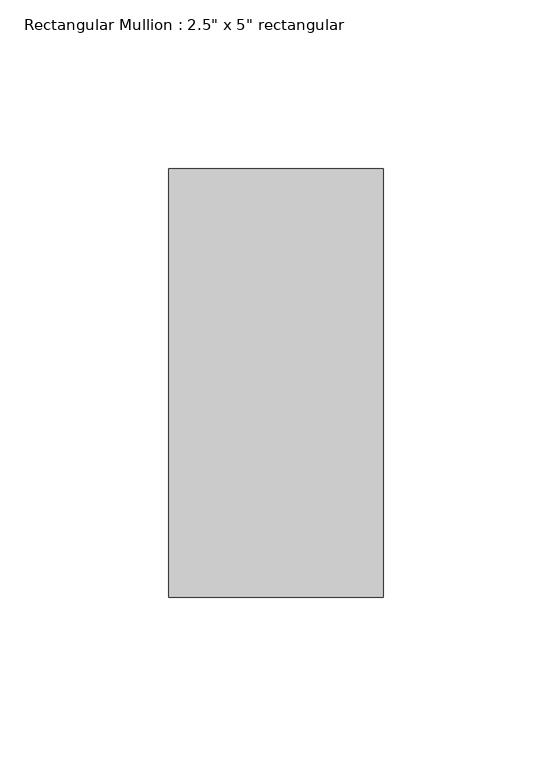
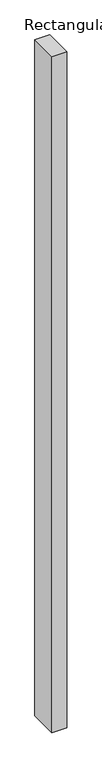
"""IFC4 building model written with IfcOpenShell, lengths in millimetres: member geometry."""

import ifcopenshell
import ifcopenshell.guid

model = None  # the IFC model being written
_history = None  # IfcOwnerHistory: only IFC2X3 demands one
_inside = {}  # id of a spatial element -> (the spatial element, [elements in it])
_under = {}  # id of a project, library or spatial element -> (it, [spatial elements below it])
_declared = {}  # id of a project -> (the project, [libraries it declares])
_typed = {}  # id of a type object -> (the type object, [elements of that type])
_made_of = {}  # id of a material, layer set ... -> (it, [elements and type objects made of it])


def new_model(schema):
    """Start an empty IFC model of exactly this schema.

    Asked for "IFC4X3", IfcOpenShell would pick the latest addendum, in which some entities
    have other attributes; the version numbers below select the first issue.
    IFC2X3 requires an IfcOwnerHistory on every rooted entity: one is made here for all.
    """
    global model, _history
    if schema == "IFC4X3":
        model = ifcopenshell.file(schema_version=(4, 3, 0, 0))
    else:
        model = ifcopenshell.file(schema=schema)
    _inside.clear()
    _under.clear()
    _declared.clear()
    _typed.clear()
    _made_of.clear()
    _history = None
    if model.schema == "IFC2X3":
        org = make("IfcOrganization", Name="unknown")
        user = make(
            "IfcPersonAndOrganization",
            ThePerson=make("IfcPerson", FamilyName="unknown"),
            TheOrganization=org,
        )
        app = make(
            "IfcApplication",
            ApplicationDeveloper=org,
            Version="unknown",
            ApplicationFullName="unknown",
            ApplicationIdentifier="unknown",
        )
        _history = make(
            "IfcOwnerHistory",
            OwningUser=user,
            OwningApplication=app,
            ChangeAction="ADDED",
            CreationDate=0,
        )
    return model


def make(cls, **values):
    """One entity of the class cls with the attributes given. An attribute that is None is left unset."""
    return model.create_entity(
        cls, **{name: value for name, value in values.items() if value is not None}
    )


def rooted(cls, **values):
    """An entity with a GlobalId (a new one), such as an element, a storey or a relation."""
    return make(cls, GlobalId=ifcopenshell.guid.new(), OwnerHistory=_history, **values)


def si_unit(unit_type, name, prefix=None):
    """IfcSIUnit, for example si_unit("LENGTHUNIT", "METRE", prefix="MILLI")."""
    return make("IfcSIUnit", UnitType=unit_type, Prefix=prefix, Name=name)


def assignment(units):
    """IfcUnitAssignment: the units of a project."""
    return None if units is None else make("IfcUnitAssignment", Units=units)


def point(xyz):
    """IfcCartesianPoint."""
    return None if xyz is None else make("IfcCartesianPoint", Coordinates=xyz)


def direction(xyz):
    """IfcDirection."""
    return None if xyz is None else make("IfcDirection", DirectionRatios=xyz)


def frame(location, z_axis=None, x_axis=None):
    """IfcAxis2Placement3D, a coordinate frame: its origin and axes. An axis left out is left unset."""
    return make(
        "IfcAxis2Placement3D",
        Location=point(location),
        Axis=direction(z_axis),
        RefDirection=direction(x_axis),
    )


def origin():
    """The frame at (0, 0, 0) with its axes left unset."""
    return frame((0.0, 0.0, 0.0))


def place(relative_to, where):
    """IfcLocalPlacement: puts the frame where relative to a parent placement (None: the world)."""
    return make(
        "IfcLocalPlacement", PlacementRelTo=relative_to, RelativePlacement=where
    )


def context(
    kind, dimensions, precision=None, world=None, true_north=None, identifier=None
):
    """IfcGeometricRepresentationContext, for example the 3D "Model" context."""
    return make(
        "IfcGeometricRepresentationContext",
        ContextIdentifier=identifier,
        ContextType=kind,
        CoordinateSpaceDimension=dimensions,
        Precision=precision,
        WorldCoordinateSystem=world,
        TrueNorth=true_north,
    )


def project(units=None, contexts=None):
    """IfcProject with its units and contexts."""
    return rooted(
        "IfcProject",
        Name="project",
        RepresentationContexts=contexts,
        UnitsInContext=assignment(units),
    )


def spatial(cls, under=None, at=None, **own):
    """A site, building, storey or space (cls), placed at a placement, below another one or the project."""
    s = rooted(cls, ObjectPlacement=at, **own)
    if under is not None:
        _under.setdefault(under.id(), (under, []))[1].append(s)
    return s


def polyline(points):
    """IfcPolyline through the points."""
    return make("IfcPolyline", Points=[point(p) for p in points])


def outline(outer, holes=None, kind="AREA"):
    """IfcArbitraryClosedProfileDef: a profile drawn as a closed curve; with holes, ...WithVoids."""
    if holes is None:
        return make("IfcArbitraryClosedProfileDef", ProfileType=kind, OuterCurve=outer)
    return make(
        "IfcArbitraryProfileDefWithVoids",
        ProfileType=kind,
        OuterCurve=outer,
        InnerCurves=holes,
    )


def extrude(swept, where, along, depth):
    """IfcExtrudedAreaSolid: the profile swept, set in the frame where, extruded along a direction by depth."""
    return make(
        "IfcExtrudedAreaSolid",
        SweptArea=swept,
        Position=where,
        ExtrudedDirection=direction(along),
        Depth=depth,
    )


def shape(context_of_items, identifier, shape_type, items):
    """IfcShapeRepresentation: the items that make up one representation, for example the "Body"."""
    return make(
        "IfcShapeRepresentation",
        ContextOfItems=context_of_items,
        RepresentationIdentifier=identifier,
        RepresentationType=shape_type,
        Items=items,
    )


def source(mapping_origin, context_of_items, identifier, shape_type, items):
    """IfcRepresentationMap: a shape defined once, which mapped items show again and again."""
    return make(
        "IfcRepresentationMap",
        MappingOrigin=mapping_origin,
        MappedRepresentation=shape(context_of_items, identifier, shape_type, items),
    )


def transform(
    local_origin,
    x_axis=None,
    y_axis=None,
    z_axis=None,
    scale=None,
    scale2=None,
    scale3=None,
    uniform=True,
):
    """IfcCartesianTransformationOperator3D, or its non-uniform kind. x_axis, y_axis, z_axis: its Axis1, 2, 3."""
    if uniform:
        return make(
            "IfcCartesianTransformationOperator3D",
            Axis1=direction(x_axis),
            Axis2=direction(y_axis),
            LocalOrigin=point(local_origin),
            Scale=scale,
            Axis3=direction(z_axis),
        )
    return make(
        "IfcCartesianTransformationOperator3DnonUniform",
        Axis1=direction(x_axis),
        Axis2=direction(y_axis),
        LocalOrigin=point(local_origin),
        Scale=scale,
        Axis3=direction(z_axis),
        Scale2=scale2,
        Scale3=scale3,
    )


def mapped(mapping_source, mapping_target):
    """IfcMappedItem: shows the shape of a source again, moved by a transform."""
    return make(
        "IfcMappedItem", MappingSource=mapping_source, MappingTarget=mapping_target
    )


def made_of(thing, what):
    """Note that an element or type object is made of a material, layer set ...; save() writes the relation."""
    if what is not None:
        _made_of.setdefault(what.id(), (what, []))[1].append(thing)
    return thing


def element(
    cls,
    number,
    at=None,
    inside=None,
    cuts=None,
    type_object=None,
    material=None,
    context=None,
    identifier="Body",
    shape_type=None,
    held_by="IfcProductDefinitionShape",
    body=None,
    shapes=None,
    **own,
):
    """One element of the class cls, such as IfcWall. Its Tag is "e" and its number.

    at: its placement. inside: the storey or other place that contains it. cuts: it is an
    opening in that element (IfcRelVoidsElement). A single representation is given by context,
    identifier, shape_type and body (its items); several are given by shapes. held_by: the class
    of the entity that holds the representations. save() writes the other relations.
    """
    e = rooted(cls, Tag="e%d" % number, ObjectPlacement=at, **own)
    if body is not None:
        shapes = [shape(context, identifier, shape_type, body)]
    if shapes is not None:
        e.Representation = make(held_by, Representations=shapes)
    if inside is not None:
        _inside.setdefault(inside.id(), (inside, []))[1].append(e)
    if cuts is not None:
        rooted(
            "IfcRelVoidsElement", RelatingBuildingElement=cuts, RelatedOpeningElement=e
        )
    if type_object is not None:
        _typed.setdefault(type_object.id(), (type_object, []))[1].append(e)
    return made_of(e, material)


def aggregate(whole, parts):
    """IfcRelAggregates: a whole, such as a stair, and the parts it consists of."""
    return rooted("IfcRelAggregates", RelatingObject=whole, RelatedObjects=parts)


def save(model, path):
    """Write the relations noted so far, then the file.

    IfcRelAggregates (storeys below a building ...), IfcRelContainedInSpatialStructure (elements
    in a storey), IfcRelDefinesByType, IfcRelAssociatesMaterial and IfcRelDeclares: one each for
    every whole, place, type object, material and project.
    """
    for whole, parts in _under.values():
        aggregate(whole, parts)
    for where, things in _inside.values():
        rooted(
            "IfcRelContainedInSpatialStructure",
            RelatedElements=things,
            RelatingStructure=where,
        )
    for kind, things in _typed.values():
        rooted("IfcRelDefinesByType", RelatedObjects=things, RelatingType=kind)
    for what, things in _made_of.values():
        rooted("IfcRelAssociatesMaterial", RelatedObjects=things, RelatingMaterial=what)
    for by, libraries in _declared.values():
        rooted("IfcRelDeclares", RelatingContext=by, RelatedDefinitions=libraries)
    model.write(path)


def member_e8b2a95c(model_context):
    return source(origin(), model_context, "Body", "SweptSolid", [
        extrude(outline(polyline([(0.0, 63.5), (0.0, -63.5), (-63.5, -63.5), (-63.5, 63.5), (0.0, 63.5)])), frame((0.0, 0.0, -3086.1), z_axis=(0.0, 0.0, 1.0), x_axis=(1.0, 0.0, 0.0)), (0.0, 0.0, 1.0), 3086.1),
    ])


if __name__ == "__main__":
    model = new_model("IFC4")
    model_context = context("Model", 3, world=origin())
    ifc_project = project(units=[si_unit("LENGTHUNIT", "METRE", prefix="MILLI")], contexts=[model_context])
    site = spatial("IfcSite", under=ifc_project)
    building = spatial("IfcBuilding", under=site)
    placement = place(None, origin())
    member_shape = member_e8b2a95c(model_context)
    element("IfcMember", 1, ObjectType="Rectangular Mullion : 2.5\" x 5\" rectangular", at=placement, inside=building, context=model_context, shape_type="MappedRepresentation", body=[
        mapped(member_shape, transform((0.0, 0.0, 0.0), x_axis=(1.0, 0.0, 0.0), y_axis=(0.0, 1.0, 0.0), z_axis=(0.0, 0.0, 1.0))),
    ])
    save(model, "model.ifc")

# Revit data of these elements
# Type "Rectangular Mullion : 2.5\" x 5\" rectangular"
#   built-in parameter 1007304 = 0.416667 (stored number, unit not read)
#   built-in parameter 1007301 = 0.104167 (stored number, unit not read)
#   built-in parameter 1007300 = 0.104167 (stored number, unit not read)
# Element 1 (IfcMember, "Rectangular Mullion : 2.5\" x 5\" rectangular")
#   Materials on its faces: "Aluminum"
# Materials
#   "Aluminum": class "Metal", colour RGB 247 247 247, transparency 0, Description = "Aluminum 6061", Cost = 0
